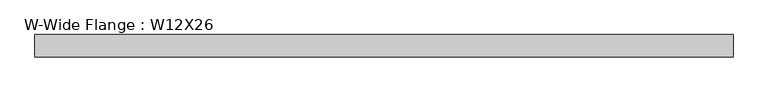
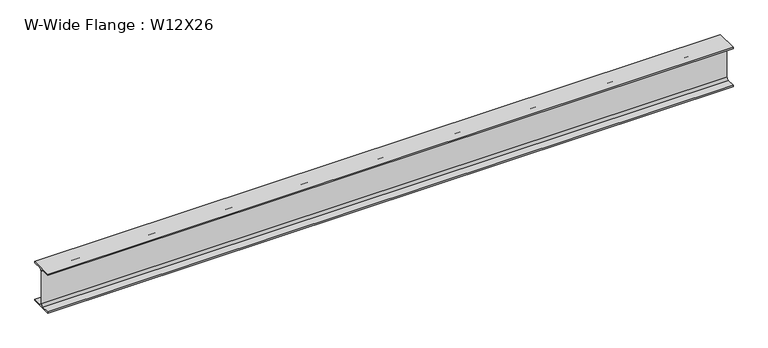
"""IFC4 building model written with IfcOpenShell, lengths in millimetres: beam geometry, W-Wide Flange : W12X26."""

from ifc_helpers import new_model, si_unit, point, frame, frame_2d, origin, place, context, project, spatial, polyline, circle_curve, trimmed, segment, composite_curve, outline, extrude, source, transform, mapped, element, save


def w_wide_flange_w12x26_a001440d(model_context):
    return source(origin(), model_context, "Body", "SweptSolid", [
        extrude(outline(composite_curve([segment(polyline([(-82.4011719, -145.5539063), (-20.2902344, -145.5539063)]), True, "CONTINUOUS"), segment(trimmed(circle_curve(frame_2d((-20.2902344, -128.190625)), 17.3632812), [point((-20.2902344, -145.5539063))], [point((-2.9269531, -128.190625))], True, "CARTESIAN"), True, "CONTINUOUS"), segment(polyline([(-2.9269531, -128.190625), (-2.9269531, 128.190625)]), True, "CONTINUOUS"), segment(trimmed(circle_curve(frame_2d((-20.2902344, 128.190625)), 17.3632812), [point((-2.9269531, 128.190625))], [point((-20.2902344, 145.5539062))], True, "CARTESIAN"), True, "CONTINUOUS"), segment(polyline([(-20.2902344, 145.5539062), (-82.4011719, 145.5539062), (-82.4011719, 155.178125), (82.4011719, 155.178125), (82.4011719, 145.5539062), (20.2902344, 145.5539062)]), True, "CONTINUOUS"), segment(trimmed(circle_curve(frame_2d((20.2902344, 128.190625)), 17.3632812), [point((20.2902344, 145.5539062))], [point((2.9269531, 128.190625))], True, "CARTESIAN"), True, "CONTINUOUS"), segment(polyline([(2.9269531, 128.190625), (2.9269531, -128.190625)]), True, "CONTINUOUS"), segment(trimmed(circle_curve(frame_2d((20.2902344, -128.190625)), 17.3632812), [point((2.9269531, -128.190625))], [point((20.2902344, -145.5539063))], True, "CARTESIAN"), True, "CONTINUOUS"), segment(polyline([(20.2902344, -145.5539063), (82.4011719, -145.5539063), (82.4011719, -155.178125), (-82.4011719, -155.178125), (-82.4011719, -145.5539063)]), True, "CONTINUOUS")], self_intersect=False)), frame((-2552.7, 0.0, 0.0), z_axis=(1.0, 0.0, 0.0), x_axis=(0.0, 1.0, 0.0)), (0.0, 0.0, 1.0), 5149.85),
    ])


if __name__ == "__main__":
    model = new_model("IFC4")
    model_context = context("Model", 3, world=origin())
    ifc_project = project(units=[si_unit("LENGTHUNIT", "METRE", prefix="MILLI")], contexts=[model_context])
    site = spatial("IfcSite", under=ifc_project)
    building = spatial("IfcBuilding", under=site)
    placement = place(None, origin())
    w_wide_flange_w12x26_shape = w_wide_flange_w12x26_a001440d(model_context)
    element("IfcBeam", 1, ObjectType="W-Wide Flange : W12X26", at=placement, inside=building, context=model_context, shape_type="MappedRepresentation", body=[
        mapped(w_wide_flange_w12x26_shape, transform((0.0, 0.0, 0.0), x_axis=(1.0, 0.0, 0.0), y_axis=(0.0, 1.0, 0.0), z_axis=(0.0, 0.0, 1.0))),
    ])
    save(model, "model.ifc")

# Revit data of these elements
# Type "W-Wide Flange : W12X26"
#   Assembly Code = "B10"
#   W = 26
#   Length [instance default] = 5' - 0"
#   bf = 0' - 6 125/256"
#   d = 1' - 0 7/32"
#   k = 0' - 1 1/16"
#   k2 = 0' - 0 175/256"
#   tf = 0' - 0 97/256"
#   tw = 0' - 0 59/256"
#   A = 0.053125 SF
#   Structural Material [instance default] = none
# Element 1 (IfcBeam, "W-Wide Flange : W12X26")
#   Structural Material = PAINTED STEEL
#   Materials on its faces: "PAINTED STEEL"
# Materials
#   "PAINTED STEEL": class "Generic", colour RGB 120 120 120, transparency 0, Cost = 0
